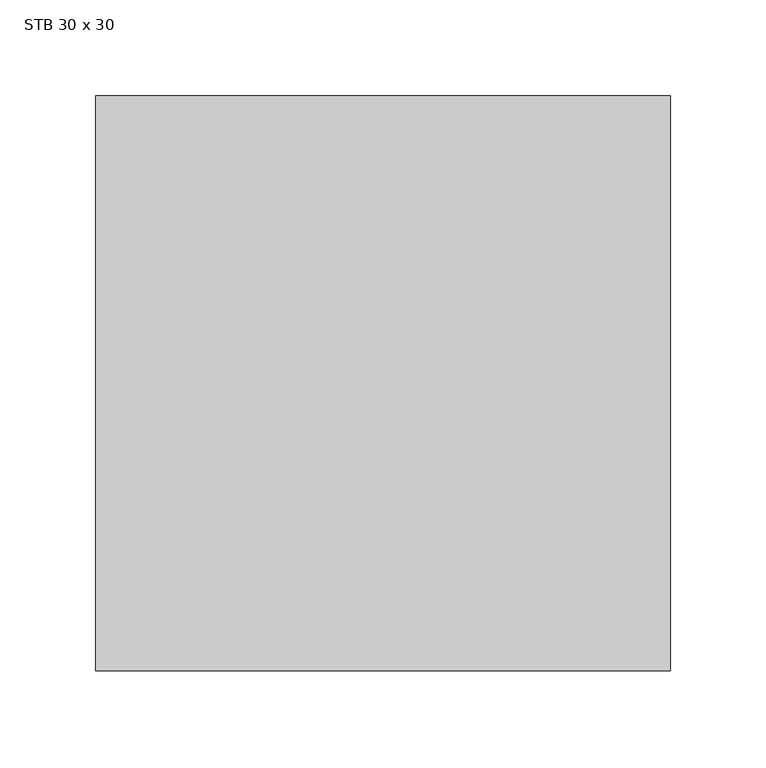
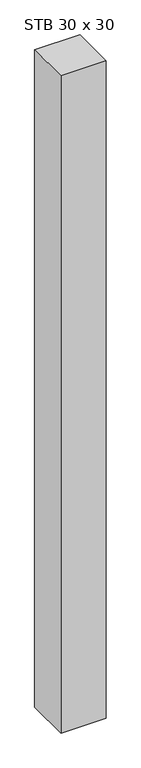
"""IFC4 building model written with IfcOpenShell, lengths in millimetres: column geometry, STB Stütze - rechteckig : STB 30 x 30."""

from ifc_helpers import new_model, si_unit, frame, origin, place, context, project, spatial, polyline, outline, extrude, source, transform, mapped, element, save


def stb_30_x_30_42b81d36(model_context):
    return source(origin(), model_context, "Body", "SweptSolid", [
        extrude(outline(polyline([(150.0, 150.0), (150.0, -150.0), (-150.0, -150.0), (-150.0, 150.0), (150.0, 150.0)])), frame((0.0, 0.0, -1580.0), z_axis=(0.0, 0.0, 1.0), x_axis=(1.0, 0.0, 0.0)), (0.0, 0.0, 1.0), 4600.0),
    ])


if __name__ == "__main__":
    model = new_model("IFC4")
    model_context = context("Model", 3, world=origin())
    ifc_project = project(units=[si_unit("LENGTHUNIT", "METRE", prefix="MILLI")], contexts=[model_context])
    site = spatial("IfcSite", under=ifc_project)
    building = spatial("IfcBuilding", under=site)
    placement = place(None, origin())
    stb_30_x_30_shape = stb_30_x_30_42b81d36(model_context)
    element("IfcColumn", 1, ObjectType="STB Stütze - rechteckig : STB 30 x 30", at=placement, inside=building, context=model_context, shape_type="MappedRepresentation", body=[
        mapped(stb_30_x_30_shape, transform((0.0, 0.0, 0.0), x_axis=(1.0, 0.0, 0.0), y_axis=(0.0, 1.0, 0.0), z_axis=(0.0, 0.0, 1.0))),
    ])
    save(model, "model.ifc")

# Revit data of these elements
# Type "STB Stütze - rechteckig : STB 30 x 30"
#   Breite = 0.300 m
#   Tiefe = 0.300 m
#   Structural Material [instance default] = Stahlbeton - Ortbeton
# Element 1 (IfcColumn, "STB Stütze - rechteckig : STB 30 x 30")
#   Materials on its faces: "Stahlbeton - Ortbeton"
# Materials
#   "Stahlbeton - Ortbeton": class "Beton", colour RGB 247 247 247, transparency 0, Cost = 0
